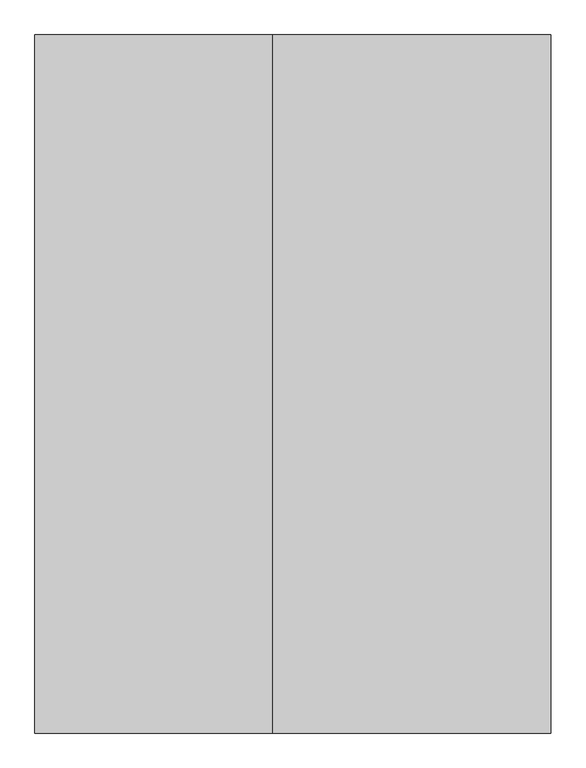
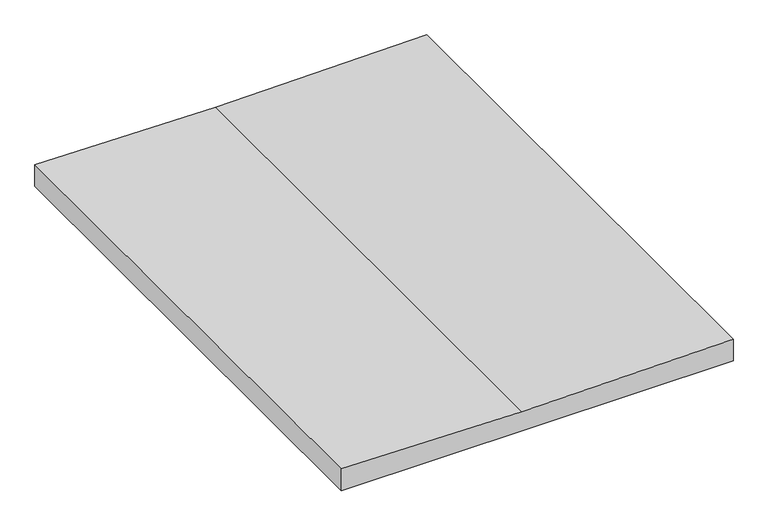
"""IFC4 building model written with IfcOpenShell, lengths in millimetres: proxy geometry, FIRESTONE INSULATION003 : FIRESTONE INSULATION003."""

import ifcopenshell
import ifcopenshell.guid

model = None  # the IFC model being written
_history = None  # IfcOwnerHistory: only IFC2X3 demands one
_inside = {}  # id of a spatial element -> (the spatial element, [elements in it])
_under = {}  # id of a project, library or spatial element -> (it, [spatial elements below it])
_declared = {}  # id of a project -> (the project, [libraries it declares])
_typed = {}  # id of a type object -> (the type object, [elements of that type])
_made_of = {}  # id of a material, layer set ... -> (it, [elements and type objects made of it])


def new_model(schema):
    """Start an empty IFC model of exactly this schema.

    Asked for "IFC4X3", IfcOpenShell would pick the latest addendum, in which some entities
    have other attributes; the version numbers below select the first issue.
    IFC2X3 requires an IfcOwnerHistory on every rooted entity: one is made here for all.
    """
    global model, _history
    if schema == "IFC4X3":
        model = ifcopenshell.file(schema_version=(4, 3, 0, 0))
    else:
        model = ifcopenshell.file(schema=schema)
    _inside.clear()
    _under.clear()
    _declared.clear()
    _typed.clear()
    _made_of.clear()
    _history = None
    if model.schema == "IFC2X3":
        org = make("IfcOrganization", Name="unknown")
        user = make(
            "IfcPersonAndOrganization",
            ThePerson=make("IfcPerson", FamilyName="unknown"),
            TheOrganization=org,
        )
        app = make(
            "IfcApplication",
            ApplicationDeveloper=org,
            Version="unknown",
            ApplicationFullName="unknown",
            ApplicationIdentifier="unknown",
        )
        _history = make(
            "IfcOwnerHistory",
            OwningUser=user,
            OwningApplication=app,
            ChangeAction="ADDED",
            CreationDate=0,
        )
    return model


def make(cls, **values):
    """One entity of the class cls with the attributes given. An attribute that is None is left unset."""
    return model.create_entity(
        cls, **{name: value for name, value in values.items() if value is not None}
    )


def rooted(cls, **values):
    """An entity with a GlobalId (a new one), such as an element, a storey or a relation."""
    return make(cls, GlobalId=ifcopenshell.guid.new(), OwnerHistory=_history, **values)


def si_unit(unit_type, name, prefix=None):
    """IfcSIUnit, for example si_unit("LENGTHUNIT", "METRE", prefix="MILLI")."""
    return make("IfcSIUnit", UnitType=unit_type, Prefix=prefix, Name=name)


def assignment(units):
    """IfcUnitAssignment: the units of a project."""
    return None if units is None else make("IfcUnitAssignment", Units=units)


def point(xyz):
    """IfcCartesianPoint."""
    return None if xyz is None else make("IfcCartesianPoint", Coordinates=xyz)


def direction(xyz):
    """IfcDirection."""
    return None if xyz is None else make("IfcDirection", DirectionRatios=xyz)


def frame(location, z_axis=None, x_axis=None):
    """IfcAxis2Placement3D, a coordinate frame: its origin and axes. An axis left out is left unset."""
    return make(
        "IfcAxis2Placement3D",
        Location=point(location),
        Axis=direction(z_axis),
        RefDirection=direction(x_axis),
    )


def origin():
    """The frame at (0, 0, 0) with its axes left unset."""
    return frame((0.0, 0.0, 0.0))


def place(relative_to, where):
    """IfcLocalPlacement: puts the frame where relative to a parent placement (None: the world)."""
    return make(
        "IfcLocalPlacement", PlacementRelTo=relative_to, RelativePlacement=where
    )


def context(
    kind, dimensions, precision=None, world=None, true_north=None, identifier=None
):
    """IfcGeometricRepresentationContext, for example the 3D "Model" context."""
    return make(
        "IfcGeometricRepresentationContext",
        ContextIdentifier=identifier,
        ContextType=kind,
        CoordinateSpaceDimension=dimensions,
        Precision=precision,
        WorldCoordinateSystem=world,
        TrueNorth=true_north,
    )


def project(units=None, contexts=None):
    """IfcProject with its units and contexts."""
    return rooted(
        "IfcProject",
        Name="project",
        RepresentationContexts=contexts,
        UnitsInContext=assignment(units),
    )


def spatial(cls, under=None, at=None, **own):
    """A site, building, storey or space (cls), placed at a placement, below another one or the project."""
    s = rooted(cls, ObjectPlacement=at, **own)
    if under is not None:
        _under.setdefault(under.id(), (under, []))[1].append(s)
    return s


def polyline(points):
    """IfcPolyline through the points."""
    return make("IfcPolyline", Points=[point(p) for p in points])


def outline(outer, holes=None, kind="AREA"):
    """IfcArbitraryClosedProfileDef: a profile drawn as a closed curve; with holes, ...WithVoids."""
    if holes is None:
        return make("IfcArbitraryClosedProfileDef", ProfileType=kind, OuterCurve=outer)
    return make(
        "IfcArbitraryProfileDefWithVoids",
        ProfileType=kind,
        OuterCurve=outer,
        InnerCurves=holes,
    )


def extrude(swept, where, along, depth):
    """IfcExtrudedAreaSolid: the profile swept, set in the frame where, extruded along a direction by depth."""
    return make(
        "IfcExtrudedAreaSolid",
        SweptArea=swept,
        Position=where,
        ExtrudedDirection=direction(along),
        Depth=depth,
    )


def shape(context_of_items, identifier, shape_type, items):
    """IfcShapeRepresentation: the items that make up one representation, for example the "Body"."""
    return make(
        "IfcShapeRepresentation",
        ContextOfItems=context_of_items,
        RepresentationIdentifier=identifier,
        RepresentationType=shape_type,
        Items=items,
    )


def source(mapping_origin, context_of_items, identifier, shape_type, items):
    """IfcRepresentationMap: a shape defined once, which mapped items show again and again."""
    return make(
        "IfcRepresentationMap",
        MappingOrigin=mapping_origin,
        MappedRepresentation=shape(context_of_items, identifier, shape_type, items),
    )


def transform(
    local_origin,
    x_axis=None,
    y_axis=None,
    z_axis=None,
    scale=None,
    scale2=None,
    scale3=None,
    uniform=True,
):
    """IfcCartesianTransformationOperator3D, or its non-uniform kind. x_axis, y_axis, z_axis: its Axis1, 2, 3."""
    if uniform:
        return make(
            "IfcCartesianTransformationOperator3D",
            Axis1=direction(x_axis),
            Axis2=direction(y_axis),
            LocalOrigin=point(local_origin),
            Scale=scale,
            Axis3=direction(z_axis),
        )
    return make(
        "IfcCartesianTransformationOperator3DnonUniform",
        Axis1=direction(x_axis),
        Axis2=direction(y_axis),
        LocalOrigin=point(local_origin),
        Scale=scale,
        Axis3=direction(z_axis),
        Scale2=scale2,
        Scale3=scale3,
    )


def mapped(mapping_source, mapping_target):
    """IfcMappedItem: shows the shape of a source again, moved by a transform."""
    return make(
        "IfcMappedItem", MappingSource=mapping_source, MappingTarget=mapping_target
    )


def made_of(thing, what):
    """Note that an element or type object is made of a material, layer set ...; save() writes the relation."""
    if what is not None:
        _made_of.setdefault(what.id(), (what, []))[1].append(thing)
    return thing


def element(
    cls,
    number,
    at=None,
    inside=None,
    cuts=None,
    type_object=None,
    material=None,
    context=None,
    identifier="Body",
    shape_type=None,
    held_by="IfcProductDefinitionShape",
    body=None,
    shapes=None,
    **own,
):
    """One element of the class cls, such as IfcWall. Its Tag is "e" and its number.

    at: its placement. inside: the storey or other place that contains it. cuts: it is an
    opening in that element (IfcRelVoidsElement). A single representation is given by context,
    identifier, shape_type and body (its items); several are given by shapes. held_by: the class
    of the entity that holds the representations. save() writes the other relations.
    """
    e = rooted(cls, Tag="e%d" % number, ObjectPlacement=at, **own)
    if body is not None:
        shapes = [shape(context, identifier, shape_type, body)]
    if shapes is not None:
        e.Representation = make(held_by, Representations=shapes)
    if inside is not None:
        _inside.setdefault(inside.id(), (inside, []))[1].append(e)
    if cuts is not None:
        rooted(
            "IfcRelVoidsElement", RelatingBuildingElement=cuts, RelatedOpeningElement=e
        )
    if type_object is not None:
        _typed.setdefault(type_object.id(), (type_object, []))[1].append(e)
    return made_of(e, material)


def aggregate(whole, parts):
    """IfcRelAggregates: a whole, such as a stair, and the parts it consists of."""
    return rooted("IfcRelAggregates", RelatingObject=whole, RelatedObjects=parts)


def save(model, path):
    """Write the relations noted so far, then the file.

    IfcRelAggregates (storeys below a building ...), IfcRelContainedInSpatialStructure (elements
    in a storey), IfcRelDefinesByType, IfcRelAssociatesMaterial and IfcRelDeclares: one each for
    every whole, place, type object, material and project.
    """
    for whole, parts in _under.values():
        aggregate(whole, parts)
    for where, things in _inside.values():
        rooted(
            "IfcRelContainedInSpatialStructure",
            RelatedElements=things,
            RelatingStructure=where,
        )
    for kind, things in _typed.values():
        rooted("IfcRelDefinesByType", RelatedObjects=things, RelatingType=kind)
    for what, things in _made_of.values():
        rooted("IfcRelAssociatesMaterial", RelatedObjects=things, RelatingMaterial=what)
    for by, libraries in _declared.values():
        rooted("IfcRelDeclares", RelatingContext=by, RelatedDefinitions=libraries)
    model.write(path)


def generic_models_44e1ce57(model_context):
    return source(origin(), model_context, "Body", "SweptSolid", [
        extrude(outline(polyline([(40131.746, -2567.3737014), (40131.746, -1090.0815411), (40218.4000089, -1090.0815411), (40208.6021556, -1886.5629484), (40218.4000089, -2567.3737014), (40131.746, -2567.3737014)])), frame((0.0, 1000.0, 0.0), z_axis=(0.0, 1.0, 0.0), x_axis=(0.0, 0.0, 1.0)), (0.0, 0.0, 1.0), 2000.0),
    ])


if __name__ == "__main__":
    model = new_model("IFC4")
    model_context = context("Model", 3, world=origin())
    ifc_project = project(units=[si_unit("LENGTHUNIT", "METRE", prefix="MILLI")], contexts=[model_context])
    site = spatial("IfcSite", under=ifc_project)
    building = spatial("IfcBuilding", under=site)
    placement = place(None, origin())
    generic_models_shape = generic_models_44e1ce57(model_context)
    element("IfcBuildingElementProxy", 1, Name="FIRESTONE INSULATION003 : FIRESTONE INSULATION003", ObjectType="FIRESTONE INSULATION003 : FIRESTONE INSULATION003", at=placement, inside=building, context=model_context, shape_type="MappedRepresentation", body=[
        mapped(generic_models_shape, transform((0.0, 0.0, 0.0), x_axis=(1.0, 0.0, 0.0), y_axis=(0.0, 1.0, 0.0), z_axis=(0.0, 0.0, 1.0))),
    ])
    save(model, "model.ifc")

# Revit data of these elements
# Type "FIRESTONE INSULATION003 : FIRESTONE INSULATION003"
#   NameOverride = "FIRESTONE INSULATION003"
# Element 1 (IfcBuildingElementProxy, "FIRESTONE INSULATION003 : FIRESTONE INSULATION003")
#   Materials on its faces: "TAPERED 2X SLEEPERS - SLOPED TO DRAIN"
# Materials
#   "TAPERED 2X SLEEPERS - SLOPED TO DRAIN": class "Unassigned", colour RGB 234 198 178, transparency 0
